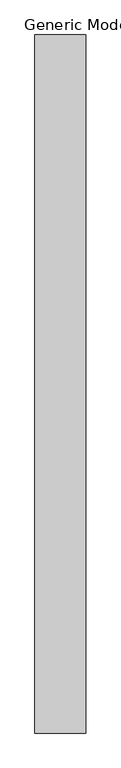
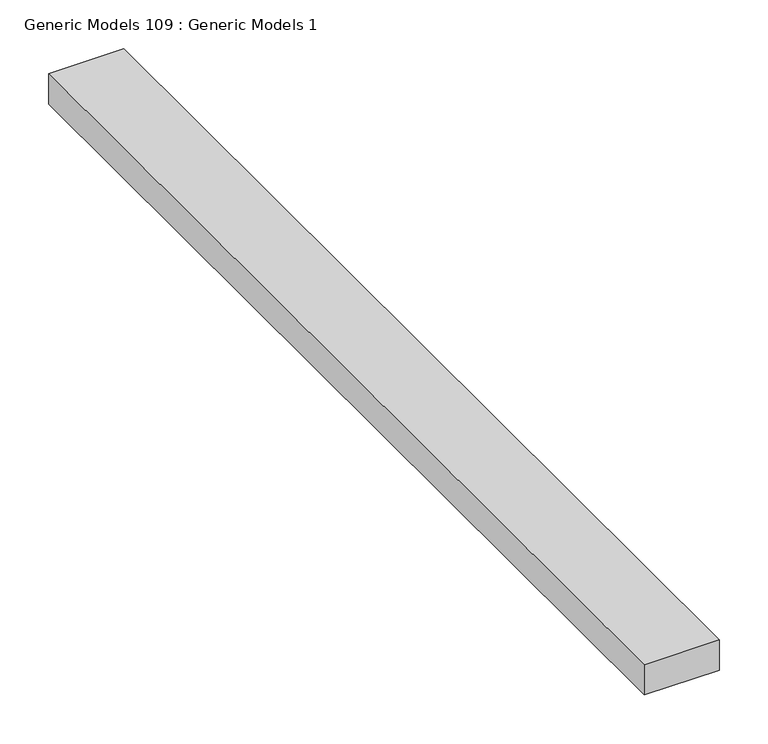
"""IFC4 building model written with IfcOpenShell, lengths in millimetres: proxy geometry, Generic Models 109 : Generic Models 1."""

from ifc_helpers import new_model, si_unit, frame, origin, place, context, project, spatial, polyline, outline, extrude, source, transform, mapped, element, save


def generic_models_109_generic_models_1_8619d77b(model_context):
    return source(origin(), model_context, "Body", "SweptSolid", [
        extrude(outline(polyline([(51003.2, 0.0), (50914.3, 0.0), (50914.3, 1219.2), (51003.2, 1219.2), (51003.2, 0.0)])), frame((0.0, 0.0, 5184.378125), z_axis=(0.0, 0.0, 1.0), x_axis=(1.0, 0.0, 0.0)), (0.0, 0.0, 1.0), 38.1),
    ])


if __name__ == "__main__":
    model = new_model("IFC4")
    model_context = context("Model", 3, world=origin())
    ifc_project = project(units=[si_unit("LENGTHUNIT", "METRE", prefix="MILLI")], contexts=[model_context])
    site = spatial("IfcSite", under=ifc_project)
    building = spatial("IfcBuilding", under=site)
    placement = place(None, origin())
    generic_models_109_generic_models_1_shape = generic_models_109_generic_models_1_8619d77b(model_context)
    element("IfcBuildingElementProxy", 1, Name="Generic Models 109 : Generic Models 1", ObjectType="Generic Models 109 : Generic Models 1", at=placement, inside=building, context=model_context, shape_type="MappedRepresentation", body=[
        mapped(generic_models_109_generic_models_1_shape, transform((0.0, 0.0, 0.0), x_axis=(1.0, 0.0, 0.0), y_axis=(0.0, 1.0, 0.0), z_axis=(0.0, 0.0, 1.0))),
    ])
    save(model, "model.ifc")

# Revit data of these elements
# Element 1 (IfcBuildingElementProxy, "Generic Models 109 : Generic Models 1")
#   Materials on its faces: "DOUBLE 2X WOOD TOP PLATE"
# Materials
#   "DOUBLE 2X WOOD TOP PLATE": class "Wood", colour RGB 234 198 147, transparency 0, Description = "Pinus Echinata", Cost = 0
